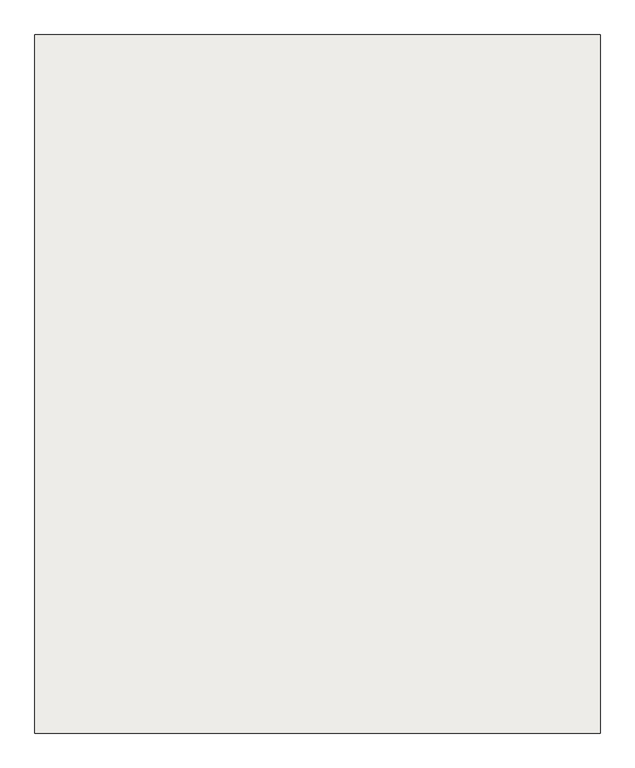
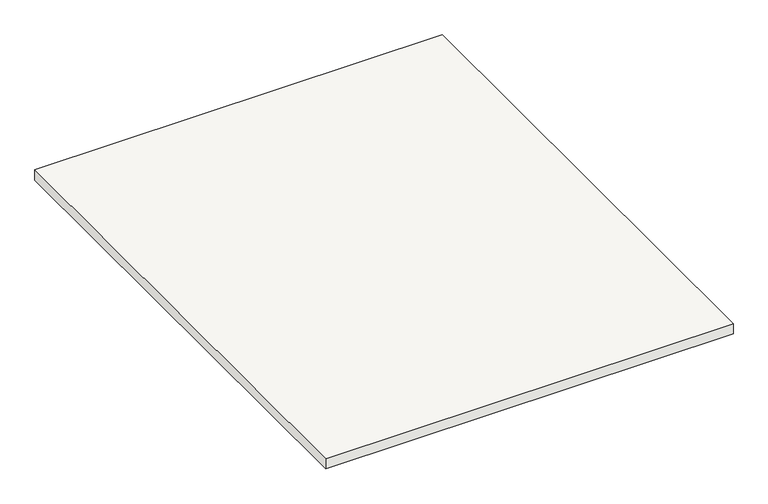
"""IFC4 building model written with IfcOpenShell, lengths in millimetres: slab geometry, Holzdecke 176 : Holzdecke 176."""

import ifcopenshell
import ifcopenshell.guid

model = None  # the IFC model being written
_history = None  # IfcOwnerHistory: only IFC2X3 demands one
_inside = {}  # id of a spatial element -> (the spatial element, [elements in it])
_under = {}  # id of a project, library or spatial element -> (it, [spatial elements below it])
_declared = {}  # id of a project -> (the project, [libraries it declares])
_typed = {}  # id of a type object -> (the type object, [elements of that type])
_made_of = {}  # id of a material, layer set ... -> (it, [elements and type objects made of it])


def new_model(schema):
    """Start an empty IFC model of exactly this schema.

    Asked for "IFC4X3", IfcOpenShell would pick the latest addendum, in which some entities
    have other attributes; the version numbers below select the first issue.
    IFC2X3 requires an IfcOwnerHistory on every rooted entity: one is made here for all.
    """
    global model, _history
    if schema == "IFC4X3":
        model = ifcopenshell.file(schema_version=(4, 3, 0, 0))
    else:
        model = ifcopenshell.file(schema=schema)
    _inside.clear()
    _under.clear()
    _declared.clear()
    _typed.clear()
    _made_of.clear()
    _history = None
    if model.schema == "IFC2X3":
        org = make("IfcOrganization", Name="unknown")
        user = make(
            "IfcPersonAndOrganization",
            ThePerson=make("IfcPerson", FamilyName="unknown"),
            TheOrganization=org,
        )
        app = make(
            "IfcApplication",
            ApplicationDeveloper=org,
            Version="unknown",
            ApplicationFullName="unknown",
            ApplicationIdentifier="unknown",
        )
        _history = make(
            "IfcOwnerHistory",
            OwningUser=user,
            OwningApplication=app,
            ChangeAction="ADDED",
            CreationDate=0,
        )
    return model


def make(cls, **values):
    """One entity of the class cls with the attributes given. An attribute that is None is left unset."""
    return model.create_entity(
        cls, **{name: value for name, value in values.items() if value is not None}
    )


def rooted(cls, **values):
    """An entity with a GlobalId (a new one), such as an element, a storey or a relation."""
    return make(cls, GlobalId=ifcopenshell.guid.new(), OwnerHistory=_history, **values)


def si_unit(unit_type, name, prefix=None):
    """IfcSIUnit, for example si_unit("LENGTHUNIT", "METRE", prefix="MILLI")."""
    return make("IfcSIUnit", UnitType=unit_type, Prefix=prefix, Name=name)


def assignment(units):
    """IfcUnitAssignment: the units of a project."""
    return None if units is None else make("IfcUnitAssignment", Units=units)


def point(xyz):
    """IfcCartesianPoint."""
    return None if xyz is None else make("IfcCartesianPoint", Coordinates=xyz)


def direction(xyz):
    """IfcDirection."""
    return None if xyz is None else make("IfcDirection", DirectionRatios=xyz)


def frame(location, z_axis=None, x_axis=None):
    """IfcAxis2Placement3D, a coordinate frame: its origin and axes. An axis left out is left unset."""
    return make(
        "IfcAxis2Placement3D",
        Location=point(location),
        Axis=direction(z_axis),
        RefDirection=direction(x_axis),
    )


def origin():
    """The frame at (0, 0, 0) with its axes left unset."""
    return frame((0.0, 0.0, 0.0))


def place(relative_to, where):
    """IfcLocalPlacement: puts the frame where relative to a parent placement (None: the world)."""
    return make(
        "IfcLocalPlacement", PlacementRelTo=relative_to, RelativePlacement=where
    )


def context(
    kind, dimensions, precision=None, world=None, true_north=None, identifier=None
):
    """IfcGeometricRepresentationContext, for example the 3D "Model" context."""
    return make(
        "IfcGeometricRepresentationContext",
        ContextIdentifier=identifier,
        ContextType=kind,
        CoordinateSpaceDimension=dimensions,
        Precision=precision,
        WorldCoordinateSystem=world,
        TrueNorth=true_north,
    )


def project(units=None, contexts=None):
    """IfcProject with its units and contexts."""
    return rooted(
        "IfcProject",
        Name="project",
        RepresentationContexts=contexts,
        UnitsInContext=assignment(units),
    )


def spatial(cls, under=None, at=None, **own):
    """A site, building, storey or space (cls), placed at a placement, below another one or the project."""
    s = rooted(cls, ObjectPlacement=at, **own)
    if under is not None:
        _under.setdefault(under.id(), (under, []))[1].append(s)
    return s


def polyline(points):
    """IfcPolyline through the points."""
    return make("IfcPolyline", Points=[point(p) for p in points])


def outline(outer, holes=None, kind="AREA"):
    """IfcArbitraryClosedProfileDef: a profile drawn as a closed curve; with holes, ...WithVoids."""
    if holes is None:
        return make("IfcArbitraryClosedProfileDef", ProfileType=kind, OuterCurve=outer)
    return make(
        "IfcArbitraryProfileDefWithVoids",
        ProfileType=kind,
        OuterCurve=outer,
        InnerCurves=holes,
    )


def extrude(swept, where, along, depth):
    """IfcExtrudedAreaSolid: the profile swept, set in the frame where, extruded along a direction by depth."""
    return make(
        "IfcExtrudedAreaSolid",
        SweptArea=swept,
        Position=where,
        ExtrudedDirection=direction(along),
        Depth=depth,
    )


def shape(context_of_items, identifier, shape_type, items):
    """IfcShapeRepresentation: the items that make up one representation, for example the "Body"."""
    return make(
        "IfcShapeRepresentation",
        ContextOfItems=context_of_items,
        RepresentationIdentifier=identifier,
        RepresentationType=shape_type,
        Items=items,
    )


def source(mapping_origin, context_of_items, identifier, shape_type, items):
    """IfcRepresentationMap: a shape defined once, which mapped items show again and again."""
    return make(
        "IfcRepresentationMap",
        MappingOrigin=mapping_origin,
        MappedRepresentation=shape(context_of_items, identifier, shape_type, items),
    )


def transform(
    local_origin,
    x_axis=None,
    y_axis=None,
    z_axis=None,
    scale=None,
    scale2=None,
    scale3=None,
    uniform=True,
):
    """IfcCartesianTransformationOperator3D, or its non-uniform kind. x_axis, y_axis, z_axis: its Axis1, 2, 3."""
    if uniform:
        return make(
            "IfcCartesianTransformationOperator3D",
            Axis1=direction(x_axis),
            Axis2=direction(y_axis),
            LocalOrigin=point(local_origin),
            Scale=scale,
            Axis3=direction(z_axis),
        )
    return make(
        "IfcCartesianTransformationOperator3DnonUniform",
        Axis1=direction(x_axis),
        Axis2=direction(y_axis),
        LocalOrigin=point(local_origin),
        Scale=scale,
        Axis3=direction(z_axis),
        Scale2=scale2,
        Scale3=scale3,
    )


def mapped(mapping_source, mapping_target):
    """IfcMappedItem: shows the shape of a source again, moved by a transform."""
    return make(
        "IfcMappedItem", MappingSource=mapping_source, MappingTarget=mapping_target
    )


def made_of(thing, what):
    """Note that an element or type object is made of a material, layer set ...; save() writes the relation."""
    if what is not None:
        _made_of.setdefault(what.id(), (what, []))[1].append(thing)
    return thing


def element(
    cls,
    number,
    at=None,
    inside=None,
    cuts=None,
    type_object=None,
    material=None,
    context=None,
    identifier="Body",
    shape_type=None,
    held_by="IfcProductDefinitionShape",
    body=None,
    shapes=None,
    **own,
):
    """One element of the class cls, such as IfcWall. Its Tag is "e" and its number.

    at: its placement. inside: the storey or other place that contains it. cuts: it is an
    opening in that element (IfcRelVoidsElement). A single representation is given by context,
    identifier, shape_type and body (its items); several are given by shapes. held_by: the class
    of the entity that holds the representations. save() writes the other relations.
    """
    e = rooted(cls, Tag="e%d" % number, ObjectPlacement=at, **own)
    if body is not None:
        shapes = [shape(context, identifier, shape_type, body)]
    if shapes is not None:
        e.Representation = make(held_by, Representations=shapes)
    if inside is not None:
        _inside.setdefault(inside.id(), (inside, []))[1].append(e)
    if cuts is not None:
        rooted(
            "IfcRelVoidsElement", RelatingBuildingElement=cuts, RelatedOpeningElement=e
        )
    if type_object is not None:
        _typed.setdefault(type_object.id(), (type_object, []))[1].append(e)
    return made_of(e, material)


def aggregate(whole, parts):
    """IfcRelAggregates: a whole, such as a stair, and the parts it consists of."""
    return rooted("IfcRelAggregates", RelatingObject=whole, RelatedObjects=parts)


def save(model, path):
    """Write the relations noted so far, then the file.

    IfcRelAggregates (storeys below a building ...), IfcRelContainedInSpatialStructure (elements
    in a storey), IfcRelDefinesByType, IfcRelAssociatesMaterial and IfcRelDeclares: one each for
    every whole, place, type object, material and project.
    """
    for whole, parts in _under.values():
        aggregate(whole, parts)
    for where, things in _inside.values():
        rooted(
            "IfcRelContainedInSpatialStructure",
            RelatedElements=things,
            RelatingStructure=where,
        )
    for kind, things in _typed.values():
        rooted("IfcRelDefinesByType", RelatedObjects=things, RelatingType=kind)
    for what, things in _made_of.values():
        rooted("IfcRelAssociatesMaterial", RelatedObjects=things, RelatingMaterial=what)
    for by, libraries in _declared.values():
        rooted("IfcRelDeclares", RelatingContext=by, RelatedDefinitions=libraries)
    model.write(path)


def slab_4f2d1623(model_context):
    return source(origin(), model_context, "Body", "SweptSolid", [
        extrude(outline(polyline([(174297.7593015, 47984.7962965), (174297.7593015, 26981.9343946), (157297.7593015, 26981.9343946), (157297.7593015, 47984.7962965), (174297.7593015, 47984.7962965)])), frame((0.0, 0.0, 2880.0), z_axis=(0.0, 0.0, 1.0), x_axis=(1.0, 0.0, 0.0)), (0.0, 0.0, 1.0), 450.0),
    ])


if __name__ == "__main__":
    model = new_model("IFC4")
    model_context = context("Model", 3, world=origin())
    ifc_project = project(units=[si_unit("LENGTHUNIT", "METRE", prefix="MILLI")], contexts=[model_context])
    site = spatial("IfcSite", under=ifc_project)
    building = spatial("IfcBuilding", under=site)
    placement = place(None, origin())
    slab_shape = slab_4f2d1623(model_context)
    element("IfcSlab", 1, ObjectType="Holzdecke 176 : Holzdecke 176", at=placement, inside=building, context=model_context, shape_type="MappedRepresentation", body=[
        mapped(slab_shape, transform((0.0, 0.0, 0.0), x_axis=(1.0, 0.0, 0.0), y_axis=(0.0, 1.0, 0.0), z_axis=(0.0, 0.0, 1.0))),
    ])
    save(model, "model.ifc")

# Revit data of these elements
# Project information
#   Organization Name = "Organization Name"
#   Organization Description = "Organization Description"
#   Building Name = "Building Name"
#   IfcOrganization = "KURIARCHITEKTEN"
#   IfcApplicationVersion = "2023.1"
#   IfcApplicationName = "Allplan"
#   IfcSite GUID = "3xMs$kp1n46ejeur8tozco"
#   IfcBuilding GUID = "0i8UyhEYT3nv9HLlo1H2X7"
#   IfcProject GUID = "2x1YFttxr4OvBiL8xtaqeA"
#   NameOverride = "GEBÄUDE 1"
#   Project Issue Date = "Issue Date"
#   Project Status = "Project Status"
#   Client Name = "Client Name"
#   Project Address = "Enter address here\nAddress Line 2"
#   Project Name = "Project Name"
#   Project Number = "Project Number"
# Type "Holzdecke 176 : Holzdecke 176"
#   Abrechnungsart = "m²"
#   Allright_Bauteil_ID = "0113De 0783954357"
#   Bezeichnung = "Holzdecke"
#   Codetext = "D-HOLZBALKEN1\\"
#   Gewerk = "Zimmer- und Holzbauarbeiten"
#   Material = "Holz"
#   Objektname = "Brettstapeldecke"
#   NameOverride = "Holzdecke"
#   Reference = "Holzdecke"
#   Status = "NEW"
#   PitchAngle = 0.00°
#   ThermalTransmittance = 0.0000 BTU/(h·ft²·°F)
#   2D Interaktion = yes
#   Combustible = no
#   Compartmentation = no
#   IsExternal = no
#   LoadBearing = yes
# Element 1 (IfcSlab, "Holzdecke 176 : Holzdecke 176")
#   Materials on its faces: "holzschalung"
# Materials
#   "holzschalung": class "Unassigned", colour RGB 128 128 128, transparency 0
